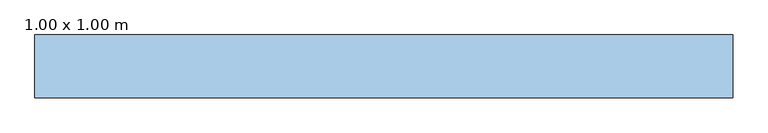
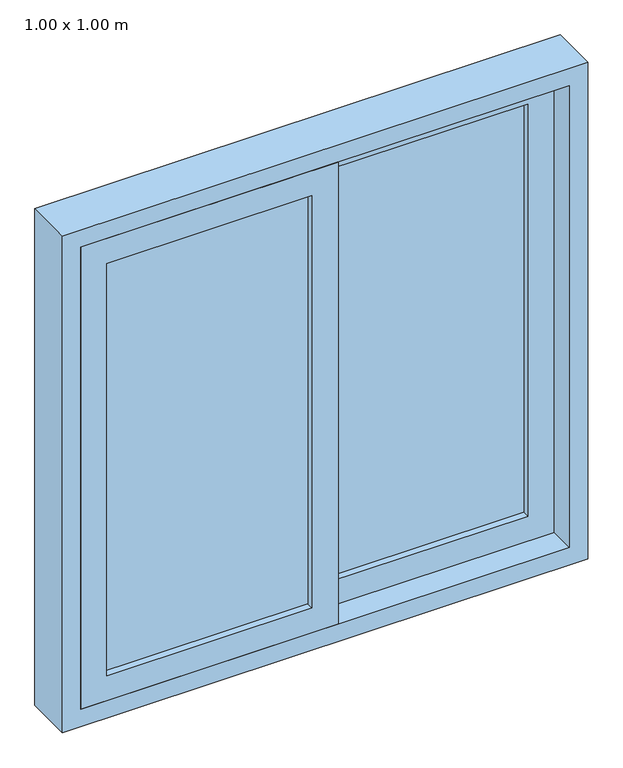
"""IFC4 building model written with IfcOpenShell, lengths in millimetres: window geometry, Janela de correr vidro - 2 Folhas : 1.00 x 1.00 m."""

import ifcopenshell
import ifcopenshell.guid

model = None  # the IFC model being written
_history = None  # IfcOwnerHistory: only IFC2X3 demands one
_inside = {}  # id of a spatial element -> (the spatial element, [elements in it])
_under = {}  # id of a project, library or spatial element -> (it, [spatial elements below it])
_declared = {}  # id of a project -> (the project, [libraries it declares])
_typed = {}  # id of a type object -> (the type object, [elements of that type])
_made_of = {}  # id of a material, layer set ... -> (it, [elements and type objects made of it])


def new_model(schema):
    """Start an empty IFC model of exactly this schema.

    Asked for "IFC4X3", IfcOpenShell would pick the latest addendum, in which some entities
    have other attributes; the version numbers below select the first issue.
    IFC2X3 requires an IfcOwnerHistory on every rooted entity: one is made here for all.
    """
    global model, _history
    if schema == "IFC4X3":
        model = ifcopenshell.file(schema_version=(4, 3, 0, 0))
    else:
        model = ifcopenshell.file(schema=schema)
    _inside.clear()
    _under.clear()
    _declared.clear()
    _typed.clear()
    _made_of.clear()
    _history = None
    if model.schema == "IFC2X3":
        org = make("IfcOrganization", Name="unknown")
        user = make(
            "IfcPersonAndOrganization",
            ThePerson=make("IfcPerson", FamilyName="unknown"),
            TheOrganization=org,
        )
        app = make(
            "IfcApplication",
            ApplicationDeveloper=org,
            Version="unknown",
            ApplicationFullName="unknown",
            ApplicationIdentifier="unknown",
        )
        _history = make(
            "IfcOwnerHistory",
            OwningUser=user,
            OwningApplication=app,
            ChangeAction="ADDED",
            CreationDate=0,
        )
    return model


def make(cls, **values):
    """One entity of the class cls with the attributes given. An attribute that is None is left unset."""
    return model.create_entity(
        cls, **{name: value for name, value in values.items() if value is not None}
    )


def rooted(cls, **values):
    """An entity with a GlobalId (a new one), such as an element, a storey or a relation."""
    return make(cls, GlobalId=ifcopenshell.guid.new(), OwnerHistory=_history, **values)


def si_unit(unit_type, name, prefix=None):
    """IfcSIUnit, for example si_unit("LENGTHUNIT", "METRE", prefix="MILLI")."""
    return make("IfcSIUnit", UnitType=unit_type, Prefix=prefix, Name=name)


def assignment(units):
    """IfcUnitAssignment: the units of a project."""
    return None if units is None else make("IfcUnitAssignment", Units=units)


def point(xyz):
    """IfcCartesianPoint."""
    return None if xyz is None else make("IfcCartesianPoint", Coordinates=xyz)


def direction(xyz):
    """IfcDirection."""
    return None if xyz is None else make("IfcDirection", DirectionRatios=xyz)


def frame(location, z_axis=None, x_axis=None):
    """IfcAxis2Placement3D, a coordinate frame: its origin and axes. An axis left out is left unset."""
    return make(
        "IfcAxis2Placement3D",
        Location=point(location),
        Axis=direction(z_axis),
        RefDirection=direction(x_axis),
    )


def origin():
    """The frame at (0, 0, 0) with its axes left unset."""
    return frame((0.0, 0.0, 0.0))


def place(relative_to, where):
    """IfcLocalPlacement: puts the frame where relative to a parent placement (None: the world)."""
    return make(
        "IfcLocalPlacement", PlacementRelTo=relative_to, RelativePlacement=where
    )


def context(
    kind, dimensions, precision=None, world=None, true_north=None, identifier=None
):
    """IfcGeometricRepresentationContext, for example the 3D "Model" context."""
    return make(
        "IfcGeometricRepresentationContext",
        ContextIdentifier=identifier,
        ContextType=kind,
        CoordinateSpaceDimension=dimensions,
        Precision=precision,
        WorldCoordinateSystem=world,
        TrueNorth=true_north,
    )


def project(units=None, contexts=None):
    """IfcProject with its units and contexts."""
    return rooted(
        "IfcProject",
        Name="project",
        RepresentationContexts=contexts,
        UnitsInContext=assignment(units),
    )


def spatial(cls, under=None, at=None, **own):
    """A site, building, storey or space (cls), placed at a placement, below another one or the project."""
    s = rooted(cls, ObjectPlacement=at, **own)
    if under is not None:
        _under.setdefault(under.id(), (under, []))[1].append(s)
    return s


def polyline(points):
    """IfcPolyline through the points."""
    return make("IfcPolyline", Points=[point(p) for p in points])


def outline(outer, holes=None, kind="AREA"):
    """IfcArbitraryClosedProfileDef: a profile drawn as a closed curve; with holes, ...WithVoids."""
    if holes is None:
        return make("IfcArbitraryClosedProfileDef", ProfileType=kind, OuterCurve=outer)
    return make(
        "IfcArbitraryProfileDefWithVoids",
        ProfileType=kind,
        OuterCurve=outer,
        InnerCurves=holes,
    )


def extrude(swept, where, along, depth):
    """IfcExtrudedAreaSolid: the profile swept, set in the frame where, extruded along a direction by depth."""
    return make(
        "IfcExtrudedAreaSolid",
        SweptArea=swept,
        Position=where,
        ExtrudedDirection=direction(along),
        Depth=depth,
    )


def shape(context_of_items, identifier, shape_type, items):
    """IfcShapeRepresentation: the items that make up one representation, for example the "Body"."""
    return make(
        "IfcShapeRepresentation",
        ContextOfItems=context_of_items,
        RepresentationIdentifier=identifier,
        RepresentationType=shape_type,
        Items=items,
    )


def source(mapping_origin, context_of_items, identifier, shape_type, items):
    """IfcRepresentationMap: a shape defined once, which mapped items show again and again."""
    return make(
        "IfcRepresentationMap",
        MappingOrigin=mapping_origin,
        MappedRepresentation=shape(context_of_items, identifier, shape_type, items),
    )


def transform(
    local_origin,
    x_axis=None,
    y_axis=None,
    z_axis=None,
    scale=None,
    scale2=None,
    scale3=None,
    uniform=True,
):
    """IfcCartesianTransformationOperator3D, or its non-uniform kind. x_axis, y_axis, z_axis: its Axis1, 2, 3."""
    if uniform:
        return make(
            "IfcCartesianTransformationOperator3D",
            Axis1=direction(x_axis),
            Axis2=direction(y_axis),
            LocalOrigin=point(local_origin),
            Scale=scale,
            Axis3=direction(z_axis),
        )
    return make(
        "IfcCartesianTransformationOperator3DnonUniform",
        Axis1=direction(x_axis),
        Axis2=direction(y_axis),
        LocalOrigin=point(local_origin),
        Scale=scale,
        Axis3=direction(z_axis),
        Scale2=scale2,
        Scale3=scale3,
    )


def mapped(mapping_source, mapping_target):
    """IfcMappedItem: shows the shape of a source again, moved by a transform."""
    return make(
        "IfcMappedItem", MappingSource=mapping_source, MappingTarget=mapping_target
    )


def made_of(thing, what):
    """Note that an element or type object is made of a material, layer set ...; save() writes the relation."""
    if what is not None:
        _made_of.setdefault(what.id(), (what, []))[1].append(thing)
    return thing


def element(
    cls,
    number,
    at=None,
    inside=None,
    cuts=None,
    type_object=None,
    material=None,
    context=None,
    identifier="Body",
    shape_type=None,
    held_by="IfcProductDefinitionShape",
    body=None,
    shapes=None,
    **own,
):
    """One element of the class cls, such as IfcWall. Its Tag is "e" and its number.

    at: its placement. inside: the storey or other place that contains it. cuts: it is an
    opening in that element (IfcRelVoidsElement). A single representation is given by context,
    identifier, shape_type and body (its items); several are given by shapes. held_by: the class
    of the entity that holds the representations. save() writes the other relations.
    """
    e = rooted(cls, Tag="e%d" % number, ObjectPlacement=at, **own)
    if body is not None:
        shapes = [shape(context, identifier, shape_type, body)]
    if shapes is not None:
        e.Representation = make(held_by, Representations=shapes)
    if inside is not None:
        _inside.setdefault(inside.id(), (inside, []))[1].append(e)
    if cuts is not None:
        rooted(
            "IfcRelVoidsElement", RelatingBuildingElement=cuts, RelatedOpeningElement=e
        )
    if type_object is not None:
        _typed.setdefault(type_object.id(), (type_object, []))[1].append(e)
    return made_of(e, material)


def aggregate(whole, parts):
    """IfcRelAggregates: a whole, such as a stair, and the parts it consists of."""
    return rooted("IfcRelAggregates", RelatingObject=whole, RelatedObjects=parts)


def save(model, path):
    """Write the relations noted so far, then the file.

    IfcRelAggregates (storeys below a building ...), IfcRelContainedInSpatialStructure (elements
    in a storey), IfcRelDefinesByType, IfcRelAssociatesMaterial and IfcRelDeclares: one each for
    every whole, place, type object, material and project.
    """
    for whole, parts in _under.values():
        aggregate(whole, parts)
    for where, things in _inside.values():
        rooted(
            "IfcRelContainedInSpatialStructure",
            RelatedElements=things,
            RelatingStructure=where,
        )
    for kind, things in _typed.values():
        rooted("IfcRelDefinesByType", RelatedObjects=things, RelatingType=kind)
    for what, things in _made_of.values():
        rooted("IfcRelAssociatesMaterial", RelatedObjects=things, RelatingMaterial=what)
    for by, libraries in _declared.values():
        rooted("IfcRelDeclares", RelatingContext=by, RelatedDefinitions=libraries)
    model.write(path)


def window_1_00_x_1_00_m_519e731f(model_context):
    return source(origin(), model_context, "Body", "SweptSolid", [
        extrude(outline(polyline([(935.0, -25.0), (935.0, 465.0), (1865.0, 465.0), (1865.0, -25.0), (935.0, -25.0)]), holes=[polyline([(1815.0, 25.0), (1815.0, 415.0), (985.0, 415.0), (985.0, 25.0), (1815.0, 25.0)])]), frame((0.0, -35.0, 0.0), z_axis=(0.0, 1.0, 0.0), x_axis=(0.0, 0.0, 1.0)), (0.0, 0.0, 1.0), 40.0),
        extrude(outline(polyline([(1865.0, 25.0), (1865.0, -465.0), (935.0, -465.0), (935.0, 25.0), (1865.0, 25.0)]), holes=[polyline([(985.0, -25.0), (985.0, -415.0), (1815.0, -415.0), (1815.0, -25.0), (985.0, -25.0)])]), frame((0.0, -85.0, 0.0), z_axis=(0.0, 1.0, 0.0), x_axis=(0.0, 0.0, 1.0)), (0.0, 0.0, 1.0), 40.0),
        extrude(outline(polyline([(1900.0, 500.0), (1900.0, -500.0), (900.0, -500.0), (900.0, 500.0), (1900.0, 500.0)]), holes=[polyline([(935.0, 465.0), (935.0, -465.0), (1865.0, -465.0), (1865.0, 465.0), (935.0, 465.0)])]), frame((0.0, -85.0, 0.0), z_axis=(0.0, 1.0, 0.0), x_axis=(0.0, 0.0, 1.0)), (0.0, 0.0, 1.0), 90.0),
        extrude(outline(polyline([(25.0, -8.0), (415.0, -8.0), (415.0, -22.0), (25.0, -22.0), (25.0, -8.0)])), frame((0.0, 0.0, 985.0), z_axis=(0.0, 0.0, 1.0), x_axis=(1.0, 0.0, 0.0)), (0.0, 0.0, 1.0), 830.0),
        extrude(outline(polyline([(-415.0, -58.0), (-25.0, -58.0), (-25.0, -72.0), (-415.0, -72.0), (-415.0, -58.0)])), frame((0.0, 0.0, 985.0), z_axis=(0.0, 0.0, 1.0), x_axis=(1.0, 0.0, 0.0)), (0.0, 0.0, 1.0), 830.0),
    ])


if __name__ == "__main__":
    model = new_model("IFC4")
    model_context = context("Model", 3, world=origin())
    ifc_project = project(units=[si_unit("LENGTHUNIT", "METRE", prefix="MILLI")], contexts=[model_context])
    site = spatial("IfcSite", under=ifc_project)
    building = spatial("IfcBuilding", under=site)
    placement = place(None, origin())
    window_1_00_x_1_00_m_shape = window_1_00_x_1_00_m_519e731f(model_context)
    element("IfcWindow", 1, ObjectType="Janela de correr vidro - 2 Folhas : 1.00 x 1.00 m", at=placement, inside=building, context=model_context, shape_type="MappedRepresentation", body=[
        mapped(window_1_00_x_1_00_m_shape, transform((0.0, 0.0, 0.0), x_axis=(1.0, 0.0, 0.0), y_axis=(0.0, 1.0, 0.0), z_axis=(0.0, 0.0, 1.0))),
    ])
    save(model, "model.ifc")

# Revit data of these elements
# Type "Janela de correr vidro - 2 Folhas : 1.00 x 1.00 m"
#   Type Mark = "J26"
#   Construction Type Id = "GSP4R"
#   Analytic Construction = "Vidraça única Pilkington 1/8 pol"
#   Visual Light Transmittance = 0.9
#   Thermal Resistance (R) = 0.271106 (m²·K)/W
#   Solar Heat Gain Coefficient = 0.78
#   Rough Width = 1.000 m
#   Rough Height = 1.000 m
#   Largura da moldura do painel = 0.050 m
#   Espessura da moldura do painel = 0.040 m
#   Height = 1.000 m
#   Heat Transfer Coefficient (U) = 3.6886 W/(m²·K)
#   Largura da estrutura = 0.035 m
#   Espessura da moldura = 0.090 m
#   Altura-padrão do peitoril = 0.900 m
#   Width = 1.000 m
#   Pingadeira = yes
#   Material da Pingadeira = Granito amarelo
#   Vidro = Vidro
#   Material da estrutura = Metal - Alumínio
#   Wall Closure = (empty or 0)
# Element 1 (IfcWindow, "Janela de correr vidro - 2 Folhas : 1.00 x 1.00 m")
#   Materials on its faces: "Metal - Alumínio", "Vidro"
# Materials
#   "Granito amarelo": class "Genérico", colour RGB 80 80 80, transparency 0, Cost = 0
#   "Vidro": class "Vidro", colour RGB 0 128 192, transparency 0.9
#   "Metal - Alumínio": class "Metal", colour RGB 247 247 247, transparency 0
